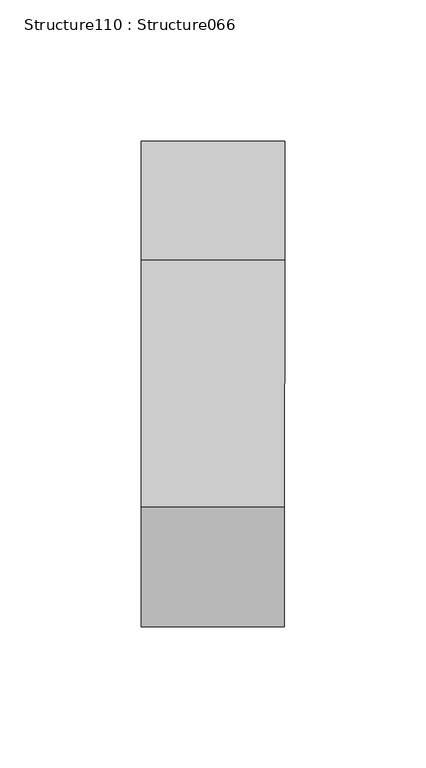
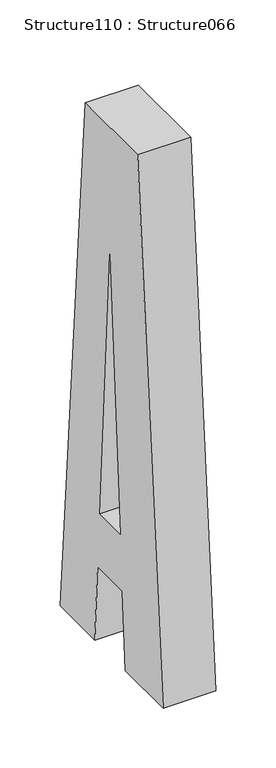
"""IFC4 building model written with IfcOpenShell, lengths in millimetres: proxy geometry, Structure110 : Structure066."""

from ifc_helpers import new_model, si_unit, frame, origin, place, context, project, spatial, polyline, outline, extrude, source, transform, mapped, element, save


def structure110_structure066_d1f14cd5(model_context):
    return source(origin(), model_context, "Body", "SweptSolid", [
        extrude(outline(polyline([(58.3911477, 0.0), (16.1366011, -537.7810299), (-71.4467402, -537.7810299), (-113.6959496, 0.0), (-50.7062387, 0.0), (-45.322746, -77.5877646), (-4.6017655, -77.5877646), (0.0, 0.0), (58.3911477, 0.0)]), holes=[polyline([(-7.6792161, -133.6760727), (-42.2492094, -133.6760727), (-24.5840236, -407.952749), (-7.6792161, -133.6760727)])]), frame((-56111.2589014, 291830.1696017, -166.7961167), z_axis=(-0.9999998917542983, 0.00046528635450596156, 0.0), x_axis=(0.00046528635450596156, 0.9999998917542983, 0.0)), (0.0, 0.0, 1.0), 50.8),
    ])


if __name__ == "__main__":
    model = new_model("IFC4")
    model_context = context("Model", 3, world=origin())
    ifc_project = project(units=[si_unit("LENGTHUNIT", "METRE", prefix="MILLI")], contexts=[model_context])
    site = spatial("IfcSite", under=ifc_project)
    building = spatial("IfcBuilding", under=site)
    placement = place(None, origin())
    structure110_structure066_shape = structure110_structure066_d1f14cd5(model_context)
    element("IfcBuildingElementProxy", 1, Name="Structure110 : Structure066", ObjectType="Structure110 : Structure066", at=placement, inside=building, context=model_context, shape_type="MappedRepresentation", body=[
        mapped(structure110_structure066_shape, transform((0.0, 0.0, 0.0), x_axis=(1.0, 0.0, 0.0), y_axis=(0.0, 1.0, 0.0), z_axis=(0.0, 0.0, 1.0))),
    ])
    save(model, "model.ifc")

# Revit data of these elements
# Type "Structure110 : Structure066"
#   NameOverride = "Structure066"
# Element 1 (IfcBuildingElementProxy, "Structure110 : Structure066")
#   Materials on its faces: "BRUSHED ALUMINUM LETTERING"
# Materials
#   "BRUSHED ALUMINUM LETTERING": class "Unassigned", colour RGB 169 181 186, transparency 0, Cost = 0
